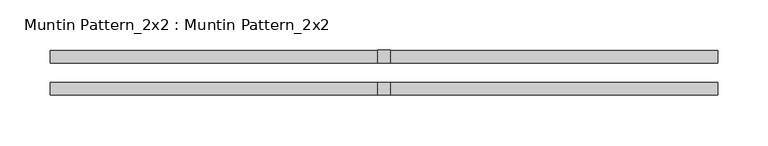
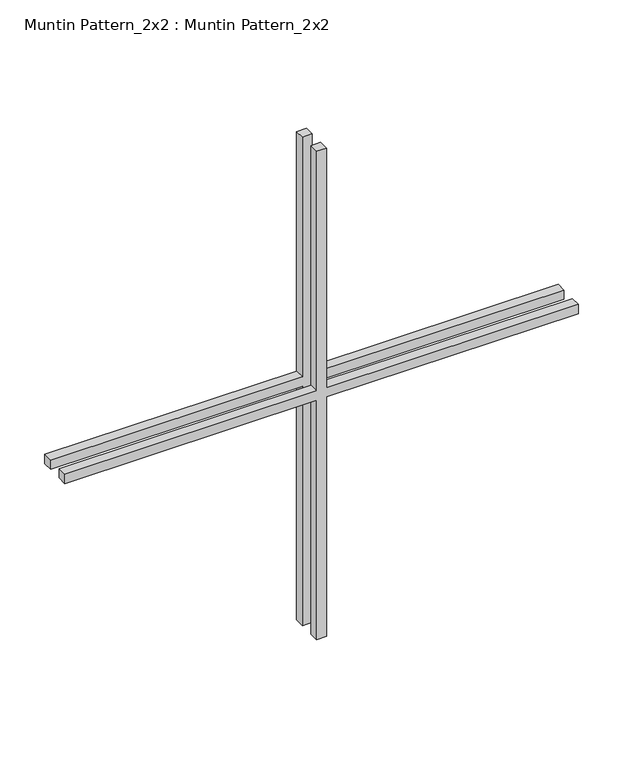
"""IFC4 building model written with IfcOpenShell, lengths in millimetres: proxy geometry, Muntin Pattern_2x2 : Muntin Pattern_2x2."""

from ifc_helpers import new_model, si_unit, frame, origin, place, context, project, spatial, polyline, outline, extrude, source, transform, mapped, element, save


def muntin_pattern_2x2_muntin_pattern_2x2_00ddd991(model_context):
    return source(origin(), model_context, "Body", "SweptSolid", [
        extrude(outline(polyline([(338.1375, -6.35), (338.1375, -330.2), (325.4375, -330.2), (325.4375, -6.35), (0.0, -6.35), (0.0, 6.35), (325.4375, 6.35), (325.4375, 330.2), (338.1375, 330.2), (338.1375, 6.35), (663.575, 6.35), (663.575, -6.35), (338.1375, -6.35)])), frame((0.0, 9.525, 0.0), z_axis=(0.0, 1.0, 0.0), x_axis=(0.0, 0.0, 1.0)), (0.0, 0.0, 1.0), 12.7),
        extrude(outline(polyline([(338.1375, -6.35), (338.1375, -330.2), (325.4375, -330.2), (325.4375, -6.35), (0.0, -6.35), (0.0, 6.35), (325.4375, 6.35), (325.4375, 330.2), (338.1375, 330.2), (338.1375, 6.35), (663.575, 6.35), (663.575, -6.35), (338.1375, -6.35)])), frame((0.0, -22.225, 0.0), z_axis=(0.0, 1.0, 0.0), x_axis=(0.0, 0.0, 1.0)), (0.0, 0.0, 1.0), 12.7),
    ])


if __name__ == "__main__":
    model = new_model("IFC4")
    model_context = context("Model", 3, world=origin())
    ifc_project = project(units=[si_unit("LENGTHUNIT", "METRE", prefix="MILLI")], contexts=[model_context])
    site = spatial("IfcSite", under=ifc_project)
    building = spatial("IfcBuilding", under=site)
    placement = place(None, origin())
    muntin_pattern_2x2_muntin_pattern_2x2_shape = muntin_pattern_2x2_muntin_pattern_2x2_00ddd991(model_context)
    element("IfcBuildingElementProxy", 1, Name="Muntin Pattern_2x2 : Muntin Pattern_2x2", ObjectType="Muntin Pattern_2x2 : Muntin Pattern_2x2", at=placement, inside=building, context=model_context, shape_type="MappedRepresentation", body=[
        mapped(muntin_pattern_2x2_muntin_pattern_2x2_shape, transform((0.0, 0.0, 0.0), x_axis=(1.0, 0.0, 0.0), y_axis=(0.0, 1.0, 0.0), z_axis=(0.0, 0.0, 1.0))),
    ])
    save(model, "model.ifc")

# Revit data of these elements
# Project information
#   Organization Name = "G3B Press"
#   Organization Description = "Paul F. Aubin Cosulting Services, Inc."
#   Building Name = "Revit Essentials for Architecture"
#   Author = "Paul F. Aubin"
#   Author Website = "https://www.paulaubin.com"
#   Copyright = "Copyright © 2020 Paul F Aubin, all rights reserved"
#   Project Issue Date = "8/1/2020"
#   Project Status = "Schematic Design"
#   Client Name = "Conceptual Underpinnings of Revit"
#   Project Address = "456 State ST\nSuite 201\nChicago, IL 60606"
#   Project Name = "Community Center"
#   Project Number = "2020.02A"
# Type "Muntin Pattern_2x2 : Muntin Pattern_2x2"
#   Width [instance default] = 4' - 0"
#   Thickness = 0' - 0 1/2"
#   Height [instance default] = 4' - 0"
#   Distance = 0' - 0 3/4"
#   Interior Material [instance default] = none
#   Exterior Material [instance default] = none
#   Default Elevation = 0
# Element 1 (IfcBuildingElementProxy, "Muntin Pattern_2x2 : Muntin Pattern_2x2")
#   Width = 2' - 2"
#   Height = 2' - 2 1/8"
#   Interior Material = Wood - Stained
#   Exterior Material = Clad - White
#   Materials on its faces: "Clad - White", "Wood - Stained"
# Materials
#   "Clad - White": class "Wood", colour RGB 242 242 238, transparency 0, Cost = 0
#   "Wood - Stained": class "Wood", colour RGB 224 178 126, transparency 0, Cost = 0
